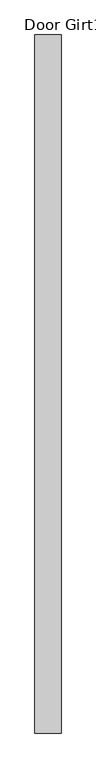
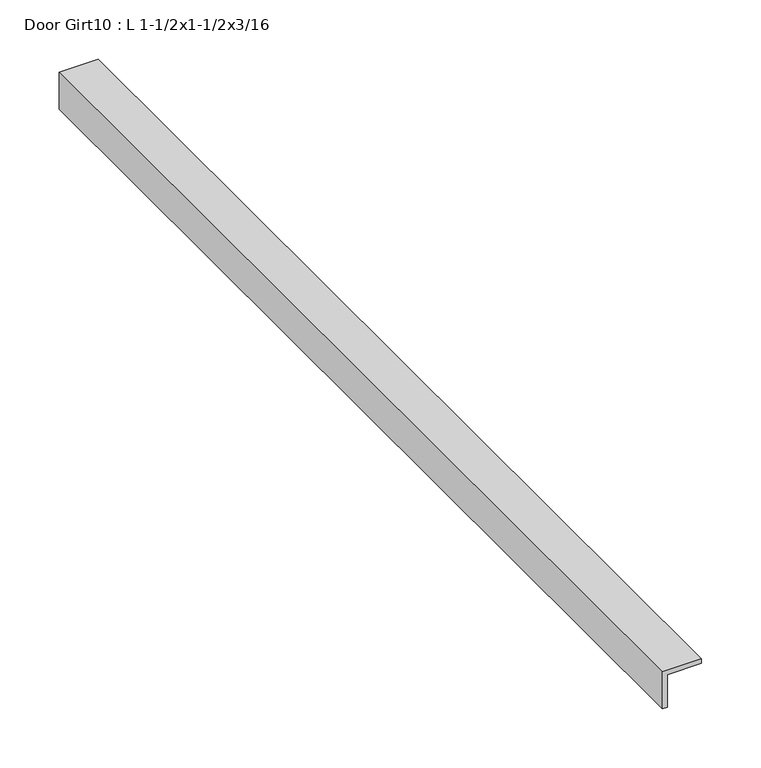
"""IFC4 building model written with IfcOpenShell, lengths in millimetres: proxy geometry, Door Girt10 : L 1-1/2x1-1/2x3/16."""

from ifc_helpers import new_model, si_unit, frame, origin, place, context, project, spatial, polyline, outline, extrude, source, transform, mapped, element, save


def door_girt10_l_1_1_2x1_1_2x3_16_4184d8b8(model_context):
    return source(origin(), model_context, "Body", "SweptSolid", [
        extrude(outline(polyline([(812.8, 587403.9934739), (812.8, 587365.8934739), (774.7, 587365.8934739), (774.7, 587370.6559739), (808.0375, 587370.6559739), (808.0375, 587403.9934739), (812.8, 587403.9934739)])), frame((0.0, -535163.4663841, 0.0), z_axis=(0.0, 1.0, 0.0), x_axis=(0.0, 0.0, 1.0)), (0.0, 0.0, 1.0), 1017.5875),
    ])


if __name__ == "__main__":
    model = new_model("IFC4")
    model_context = context("Model", 3, world=origin())
    ifc_project = project(units=[si_unit("LENGTHUNIT", "METRE", prefix="MILLI")], contexts=[model_context])
    site = spatial("IfcSite", under=ifc_project)
    building = spatial("IfcBuilding", under=site)
    placement = place(None, origin())
    door_girt10_l_1_1_2x1_1_2x3_16_shape = door_girt10_l_1_1_2x1_1_2x3_16_4184d8b8(model_context)
    element("IfcBuildingElementProxy", 1, Name="Door Girt10 : L 1-1/2x1-1/2x3/16", ObjectType="Door Girt10 : L 1-1/2x1-1/2x3/16", at=placement, inside=building, context=model_context, shape_type="MappedRepresentation", body=[
        mapped(door_girt10_l_1_1_2x1_1_2x3_16_shape, transform((0.0, 0.0, 0.0), x_axis=(1.0, 0.0, 0.0), y_axis=(0.0, 1.0, 0.0), z_axis=(0.0, 0.0, 1.0))),
    ])
    save(model, "model.ifc")

# Revit data of these elements
# Element 1 (IfcBuildingElementProxy, "Door Girt10 : L 1-1/2x1-1/2x3/16")
#   Materials on its faces: "1-1/2\"X1-1/2\" GALV. STL L"
# Materials
#   "1-1/2\"X1-1/2\" GALV. STL L": class "Generic", colour RGB 211 211 207, transparency 0, Cost = 0
